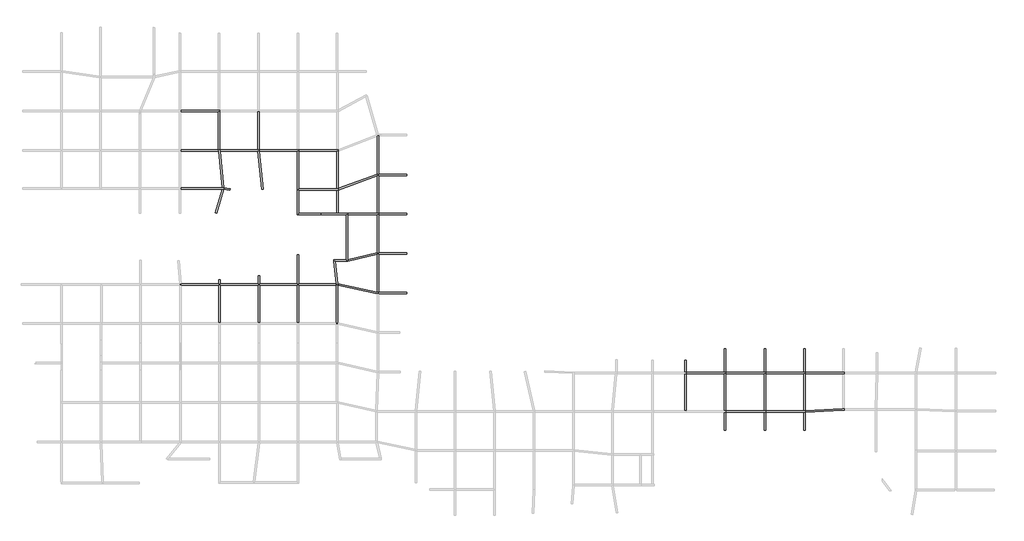
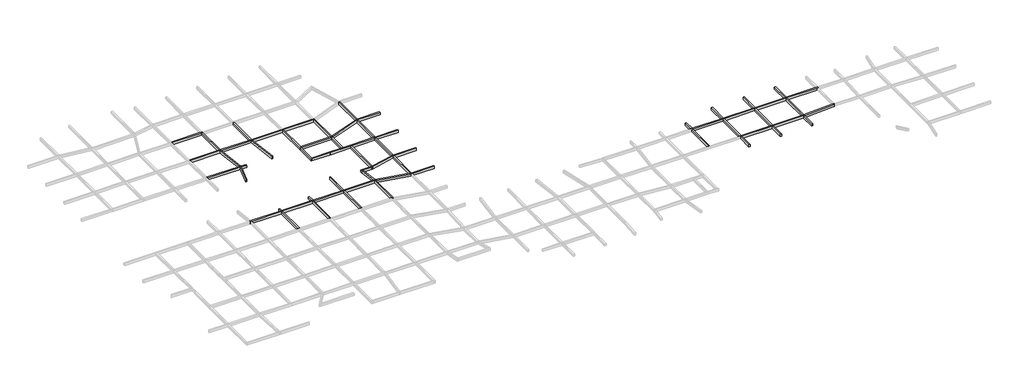
# One storey, part 5 of 8: 63 beams.
"""IFC4 building model written with IfcOpenShell, lengths in millimetres."""

from ifc_helpers import new_model, si_unit, frame, origin, place, context, project, spatial, polyline, outline, extrude, faceted_brep, element, save

model = new_model("IFC4")

# Units and contexts
model_context = context("Model", 3, world=origin())
ifc_project = project(units=[si_unit("LENGTHUNIT", "METRE", prefix="MILLI")], contexts=[model_context])

# Site, building, storey
site = spatial("IfcSite", under=ifc_project)
building = spatial("IfcBuilding", under=site)
storey = spatial("IfcBuildingStorey", under=building, Name="层高", Elevation=3300.0)

# Beams
placement = place(None, origin())
element("IfcBeam", 1, ObjectType="混凝土 - 矩形梁 : KL_beam", at=placement, inside=storey, context=model_context, shape_type="Brep", body=[
    faceted_brep([(134334.403154, 87731.7102801, 3300.0), (134334.403154, 88015.281938, 3300.0), (134334.403154, 88031.7102801, 3300.0), (134032.8693125, 88031.7102801, 3300.0), (125748.8238729, 88031.7102801, 3300.0), (125748.8238729, 87731.7102801, 3300.0), (133999.7671497, 87731.7102801, 3300.0), (134189.0731521, 87731.7102801, 3300.0), (134334.403154, 87731.7102801, 2700.0), (125748.8238729, 87731.7102801, 2700.0), (133999.7671497, 87731.7102801, 2700.0), (134189.0731521, 87731.7102801, 2700.0), (134334.403154, 88031.7102801, 2700.0), (134334.403154, 88015.281938, 2700.0), (125748.8238729, 88031.7102801, 2700.0), (134032.8693125, 88031.7102801, 2700.0)], [[[0, 1, 2, 3, 4, 5, 6, 7]], [[8, 0, 7, 6, 5, 9, 10, 11]], [[12, 13, 8, 11, 10, 9, 14, 15]], [[2, 12, 15, 14, 4, 3]], [[5, 4, 14, 9]], [[2, 1, 0, 8, 13, 12]]]),
])
element("IfcBeam", 2, ObjectType="混凝土 - 矩形梁 : KL_beam", at=placement, inside=storey, context=model_context, shape_type="Brep", body=[
    faceted_brep([(133564.8960768, 95631.7102801, 3300.0), (133548.8238805, 95631.7102801, 3300.0), (133263.3622352, 95631.7102801, 3300.0), (133293.7375146, 95331.7102801, 3300.0), (134032.8693125, 88031.7102801, 3300.0), (134334.403154, 88031.7102801, 3300.0), (133595.2713562, 95331.7102801, 3300.0), (133263.3622352, 95631.7102801, 2700.0), (133293.7375146, 95331.7102801, 2700.0), (134032.8693125, 88031.7102801, 2700.0), (133548.8238805, 95631.7102801, 2700.0), (133564.8960768, 95631.7102801, 2700.0), (133595.2713562, 95331.7102801, 2700.0), (134334.403154, 88031.7102801, 2700.0)], [[[0, 1, 2, 3, 4, 5, 6]], [[2, 7, 8, 9, 4, 3]], [[7, 10, 11, 12, 13, 9, 8]], [[11, 0, 6, 5, 13, 12]], [[5, 4, 9, 13]], [[2, 1, 0, 11, 10, 7]]]),
])
element("IfcBeam", 3, ObjectType="混凝土 - 矩形梁 : KL_beam", at=placement, inside=storey, context=model_context, shape_type="Brep", body=[
    faceted_brep([(125748.8238728, 95631.7102801, 3300.0), (125748.8238728, 95331.7102801, 3300.0), (133293.7375146, 95331.7102801, 3300.0), (133263.3622352, 95631.7102801, 3300.0), (133248.8238805, 95631.7102801, 3300.0), (125748.8238728, 95331.7102801, 2700.0), (133293.7375146, 95331.7102801, 2700.0), (125748.8238728, 95631.7102801, 2700.0), (133248.8238805, 95631.7102801, 2700.0), (133263.3622352, 95631.7102801, 2700.0)], [[[0, 1, 2, 3, 4]], [[1, 5, 6, 2]], [[5, 7, 8, 9, 6]], [[7, 0, 4, 3, 9, 8]], [[1, 0, 7, 5]], [[3, 2, 6, 9]]]),
])
element("IfcBeam", 4, ObjectType="混凝土 - 矩形梁 : KL_beam", at=placement, inside=storey, context=model_context, shape_type="Brep", body=[
    faceted_brep([(133548.8238805, 103231.7102801, 3300.0), (133548.8238805, 103531.7102801, 3300.0), (133248.8238805, 103531.7102801, 3300.0), (125748.8238726, 103531.7102801, 3300.0), (125748.8238726, 103231.7102801, 3300.0), (133248.8238805, 103231.7102801, 3300.0), (133548.8238805, 103231.7102801, 2700.0), (125748.8238726, 103231.7102801, 2700.0), (133248.8238805, 103231.7102801, 2700.0), (133548.8238805, 103531.7102801, 2700.0), (125748.8238726, 103531.7102801, 2700.0), (133248.8238805, 103531.7102801, 2700.0)], [[[0, 1, 2, 3, 4, 5]], [[6, 0, 5, 4, 7, 8]], [[9, 6, 8, 7, 10, 11]], [[1, 9, 11, 10, 3, 2]], [[4, 3, 10, 7]], [[1, 0, 6, 9]]]),
])
element("IfcBeam", 5, ObjectType="混凝土 - 矩形梁 : KL_beam", at=placement, inside=storey, context=model_context, shape_type="Brep", body=[
    faceted_brep([(133548.8238805, 103231.7102801, 3300.0), (133248.8238805, 103231.7102801, 3300.0), (133248.8238805, 95631.7102801, 3300.0), (133263.3622352, 95631.7102801, 3300.0), (133548.8238805, 95631.7102801, 3300.0), (133248.8238805, 103231.7102801, 2700.0), (133248.8238805, 95631.7102801, 2700.0), (133548.8238805, 103231.7102801, 2700.0), (133548.8238805, 95631.7102801, 2700.0), (133263.3622352, 95631.7102801, 2700.0)], [[[0, 1, 2, 3, 4]], [[1, 5, 6, 2]], [[5, 7, 8, 9, 6]], [[7, 0, 4, 8]], [[1, 0, 7, 5]], [[4, 3, 2, 6, 9, 8]]]),
])
element("IfcBeam", 6, ObjectType="混凝土 - 矩形梁 : KL_beam", at=placement, inside=storey, context=model_context, shape_type="Brep", body=[
    faceted_brep([(133564.8960768, 95631.7102801, 3300.0), (133595.2713562, 95331.7102801, 3300.0), (141163.7632738, 95331.7102801, 3300.0), (141465.4157577, 95331.7102801, 3300.0), (141448.8238805, 95489.571447, 3300.0), (141433.8844871, 95631.7102801, 3300.0), (141148.8238805, 95631.7102801, 3300.0), (133595.2713562, 95331.7102801, 2700.0), (141163.7632738, 95331.7102801, 2700.0), (141465.4157577, 95331.7102801, 2700.0), (133564.8960768, 95631.7102801, 2700.0), (141148.8238805, 95631.7102801, 2700.0), (141433.8844871, 95631.7102801, 2700.0), (141448.8238805, 95489.571447, 2700.0)], [[[0, 1, 2, 3, 4, 5, 6]], [[1, 7, 8, 9, 3, 2]], [[7, 10, 11, 12, 13, 9, 8]], [[10, 0, 6, 5, 12, 11]], [[1, 0, 10, 7]], [[5, 4, 3, 9, 13, 12]]]),
])
element("IfcBeam", 7, ObjectType="混凝土 - 矩形梁 : KL_beam", at=placement, inside=storey, context=model_context, shape_type="Brep", body=[
    faceted_brep([(135608.9251063, 87848.8786772, 3300.0), (135570.0863411, 87551.4033835, 3300.0), (135570.0863411, 87551.4033835, 2700.0), (135608.9251063, 87848.8786772, 2700.0), (134334.403154, 88015.281938, 3300.0), (134334.403154, 87731.7102801, 3300.0), (134189.0731521, 87731.7102801, 3300.0), (134307.4261, 87716.2579637, 3300.0), (134189.0731521, 87731.7102801, 2700.0), (134307.4261, 87716.2579637, 2700.0), (134334.403154, 87731.7102801, 2700.0), (134334.403154, 88015.281938, 2700.0)], [[[0, 1, 2, 3]], [[1, 0, 4, 5, 6, 7]], [[2, 1, 7, 6, 8, 9]], [[3, 2, 9, 8, 10, 11]], [[0, 3, 11, 4]], [[5, 10, 8, 6]], [[10, 5, 4, 11]]]),
])
element("IfcBeam", 8, ObjectType="混凝土 - 矩形梁 : KL_beam", at=placement, inside=storey, context=model_context, shape_type="SweptSolid", body=[
    extrude(outline(polyline([(142263.3241783, 87740.1187657), (141964.9676097, 87708.7602268), (141163.7632738, 95331.7102801), (141465.4157577, 95331.7102801), (142263.3241783, 87740.1187657)])), frame((0.0, 0.0, 2700.0), z_axis=(0.0, 0.0, 1.0), x_axis=(1.0, 0.0, 0.0)), (0.0, 0.0, 1.0), 600.0),
])
element("IfcBeam", 9, ObjectType="混凝土 - 矩形梁 : KL_beam", at=placement, inside=storey, context=model_context, shape_type="Brep", body=[
    faceted_brep([(132928.4176001, 82907.0838029, 3300.0), (132640.0390913, 82989.7750097, 3300.0), (132640.0390913, 82989.7750097, 2700.0), (132928.4176001, 82907.0838029, 2700.0), (134307.4261, 87716.2579637, 3300.0), (134189.0731521, 87731.7102801, 3300.0), (134063.2445918, 87731.7102801, 3300.0), (133999.7671497, 87731.7102801, 3300.0), (133999.7671497, 87731.7102801, 2700.0), (134063.2445918, 87731.7102801, 2700.0), (134189.0731521, 87731.7102801, 2700.0), (134307.4261, 87716.2579637, 2700.0)], [[[0, 1, 2, 3]], [[1, 0, 4, 5, 6, 7]], [[2, 1, 7, 8]], [[3, 2, 8, 9, 10, 11]], [[0, 3, 11, 4]], [[8, 7, 6, 5, 10, 9]], [[5, 4, 11, 10]]]),
])
element("IfcBeam", 10, ObjectType="混凝土 - 矩形梁 : KL_beam", at=placement, inside=storey, context=model_context, shape_type="Brep", body=[
    faceted_brep([(141448.8238805, 103231.7102801, 3300.0), (141148.8238805, 103231.7102801, 3300.0), (141148.8238805, 95631.7102801, 3300.0), (141433.8844871, 95631.7102801, 3300.0), (141448.8238805, 95489.571447, 3300.0), (141448.8238805, 95631.7102801, 3300.0), (141148.8238805, 103231.7102801, 2700.0), (141148.8238805, 95631.7102801, 2700.0), (141448.8238805, 103231.7102801, 2700.0), (141448.8238805, 95631.7102801, 2700.0), (141448.8238805, 95489.571447, 2700.0), (141433.8844871, 95631.7102801, 2700.0)], [[[0, 1, 2, 3, 4, 5]], [[1, 6, 7, 2]], [[6, 8, 9, 10, 11, 7]], [[8, 0, 5, 4, 10, 9]], [[1, 0, 8, 6]], [[11, 3, 2, 7]], [[3, 11, 10, 4]]]),
])
element("IfcBeam", 11, ObjectType="混凝土 - 矩形梁 : KL_beam", at=placement, inside=storey, context=model_context, shape_type="Brep", body=[
    faceted_brep([(149348.8238805, 95331.7102801, 3300.0), (149348.8238805, 95631.7102801, 3300.0), (149048.8238805, 95631.7102801, 3300.0), (141448.8238805, 95631.7102801, 3300.0), (141448.8238805, 95489.571447, 3300.0), (141465.4157577, 95331.7102801, 3300.0), (149048.8238805, 95331.7102801, 3300.0), (141465.4157577, 95331.7102801, 2700.0), (149048.8238805, 95331.7102801, 2700.0), (149348.8238805, 95331.7102801, 2700.0), (149348.8238805, 95631.7102801, 2700.0), (141448.8238805, 95489.571447, 2700.0), (141448.8238805, 95631.7102801, 2700.0), (149048.8238805, 95631.7102801, 2700.0)], [[[0, 1, 2, 3, 4, 5, 6]], [[5, 7, 8, 9, 0, 6]], [[10, 9, 8, 7, 11, 12, 13]], [[1, 10, 13, 12, 3, 2]], [[7, 5, 4, 11]], [[4, 3, 12, 11]], [[1, 0, 9, 10]]]),
])
element("IfcBeam", 12, ObjectType="混凝土 - 矩形梁 : KL_beam", at=placement, inside=storey, context=model_context, shape_type="Brep", body=[
    faceted_brep([(149048.8238805, 87550.0782767, 3300.0), (149348.8238805, 87550.0782767, 3300.0), (149348.8238805, 87850.0782767, 3300.0), (149348.8238805, 95331.7102801, 3300.0), (149048.8238805, 95331.7102801, 3300.0), (149048.8238805, 87550.0782767, 2700.0), (149048.8238805, 95331.7102801, 2700.0), (149348.8238805, 87550.0782767, 2700.0), (149348.8238805, 95331.7102801, 2700.0), (149348.8238805, 87850.0782767, 2700.0)], [[[0, 1, 2, 3, 4]], [[5, 0, 4, 6]], [[7, 5, 6, 8, 9]], [[1, 7, 9, 8, 3, 2]], [[4, 3, 8, 6]], [[1, 0, 5, 7]]]),
])
element("IfcBeam", 13, ObjectType="混凝土 - 矩形梁 : KL_beam", at=placement, inside=storey, context=model_context, shape_type="Brep", body=[
    faceted_brep([(157248.8238805, 95331.7102801, 3300.0), (157248.8238805, 95378.6181363, 3300.0), (157248.8238805, 95631.7102801, 3300.0), (156948.8238805, 95631.7102801, 3300.0), (149348.8238805, 95631.7102801, 3300.0), (149348.8238805, 95331.7102801, 3300.0), (156948.8238805, 95331.7102801, 3300.0), (157248.8238805, 95331.7102801, 2700.0), (149348.8238805, 95331.7102801, 2700.0), (156948.8238805, 95331.7102801, 2700.0), (157248.8238805, 95631.7102801, 2700.0), (157248.8238805, 95378.6181363, 2700.0), (149348.8238805, 95631.7102801, 2700.0), (156948.8238805, 95631.7102801, 2700.0)], [[[0, 1, 2, 3, 4, 5, 6]], [[7, 0, 6, 5, 8, 9]], [[10, 11, 7, 9, 8, 12, 13]], [[2, 10, 13, 12, 4, 3]], [[5, 4, 12, 8]], [[2, 1, 0, 7, 11, 10]]]),
])
element("IfcBeam", 14, ObjectType="混凝土 - 矩形梁 : KL_beam", at=placement, inside=storey, context=model_context, shape_type="Brep", body=[
    faceted_brep([(157248.8238805, 87550.0782767, 3300.0), (157248.8238805, 87595.0471459, 3300.0), (157248.8238805, 87850.0782767, 3300.0), (156948.8238805, 87850.0782767, 3300.0), (149348.8238805, 87850.0782767, 3300.0), (149348.8238805, 87550.0782767, 3300.0), (156948.8238805, 87550.0782767, 3300.0), (157248.8238805, 87550.0782767, 2700.0), (149348.8238805, 87550.0782767, 2700.0), (156948.8238805, 87550.0782767, 2700.0), (157248.8238805, 87850.0782767, 2700.0), (157248.8238805, 87595.0471459, 2700.0), (149348.8238805, 87850.0782767, 2700.0), (156948.8238805, 87850.0782767, 2700.0)], [[[0, 1, 2, 3, 4, 5, 6]], [[7, 0, 6, 5, 8, 9]], [[10, 11, 7, 9, 8, 12, 13]], [[2, 10, 13, 12, 4, 3]], [[5, 4, 12, 8]], [[2, 1, 0, 7, 11, 10]]]),
])
element("IfcBeam", 15, ObjectType="混凝土 - 矩形梁 : KL_beam", at=placement, inside=storey, context=model_context, shape_type="Brep", body=[
    faceted_brep([(157248.8238805, 95331.7102801, 3300.0), (156948.8238805, 95331.7102801, 3300.0), (156948.8238805, 87850.0782767, 3300.0), (157248.8238805, 87850.0782767, 3300.0), (157248.8238805, 87914.3004777, 3300.0), (156948.8238805, 95331.7102801, 2700.0), (156948.8238805, 87850.0782767, 2700.0), (157248.8238805, 95331.7102801, 2700.0), (157248.8238805, 87914.3004777, 2700.0), (157248.8238805, 87850.0782767, 2700.0)], [[[0, 1, 2, 3, 4]], [[1, 5, 6, 2]], [[5, 7, 8, 9, 6]], [[7, 0, 4, 3, 9, 8]], [[1, 0, 7, 5]], [[3, 2, 6, 9]]]),
])
element("IfcBeam", 16, ObjectType="混凝土 - 矩形梁 : KL_beam", at=placement, inside=storey, context=model_context, shape_type="Brep", body=[
    faceted_brep([(149048.8238805, 82650.0782767, 3300.0), (149348.8238805, 82650.0782767, 3300.0), (149348.8238805, 82950.0782767, 3300.0), (149348.8238805, 87550.0782767, 3300.0), (149048.8238805, 87550.0782767, 3300.0), (149048.8238805, 82650.0782767, 2700.0), (149048.8238805, 87550.0782767, 2700.0), (149348.8238805, 82650.0782767, 2700.0), (149348.8238805, 87550.0782767, 2700.0), (149348.8238805, 82950.0782767, 2700.0)], [[[0, 1, 2, 3, 4]], [[5, 0, 4, 6]], [[7, 5, 6, 8, 9]], [[1, 7, 9, 8, 3, 2]], [[4, 3, 8, 6]], [[1, 0, 5, 7]]]),
])
element("IfcBeam", 17, ObjectType="混凝土 - 矩形梁 : KL_beam", at=placement, inside=storey, context=model_context, shape_type="SweptSolid", body=[
    extrude(outline(polyline([(153790.5556896, 82950.0782767), (153790.5556896, 82650.0782767), (149348.8238805, 82650.0782767), (149348.8238805, 82950.0782767), (153790.5556896, 82950.0782767)])), frame((0.0, 0.0, 2700.0), z_axis=(0.0, 0.0, 1.0), x_axis=(1.0, 0.0, 0.0)), (0.0, 0.0, 1.0), 600.0),
])
element("IfcBeam", 18, ObjectType="混凝土 - 矩形梁 : KL_beam", at=placement, inside=storey, context=model_context, shape_type="Brep", body=[
    faceted_brep([(153790.5556896, 82950.0782767, 3300.0), (153790.5556896, 82650.0782767, 3300.0), (158923.8473255, 82650.0782767, 3300.0), (159223.8473255, 82650.0782767, 3300.0), (159223.8473255, 82950.0782767, 3300.0), (157248.8238805, 82950.0782767, 3300.0), (156948.8238805, 82950.0782767, 3300.0), (153790.5556896, 82650.0782767, 2700.0), (158923.8473255, 82650.0782767, 2700.0), (159223.8473255, 82650.0782767, 2700.0), (153790.5556896, 82950.0782767, 2700.0), (156948.8238805, 82950.0782767, 2700.0), (157248.8238805, 82950.0782767, 2700.0), (159223.8473255, 82950.0782767, 2700.0)], [[[0, 1, 2, 3, 4, 5, 6]], [[1, 7, 8, 9, 3, 2]], [[7, 10, 11, 12, 13, 9, 8]], [[10, 0, 6, 5, 4, 13, 12, 11]], [[0, 10, 7, 1]], [[4, 3, 9, 13]]]),
])
element("IfcBeam", 19, ObjectType="混凝土 - 矩形梁 : KL_beam", at=placement, inside=storey, context=model_context, shape_type="SweptSolid", body=[
    extrude(outline(polyline([(156948.8238805, 87550.0782767), (157248.8238805, 87550.0782767), (157248.8238805, 82950.0782767), (156948.8238805, 82950.0782767), (156948.8238805, 87550.0782767)])), frame((0.0, 0.0, 2700.0), z_axis=(0.0, 0.0, 1.0), x_axis=(1.0, 0.0, 0.0)), (0.0, 0.0, 1.0), 600.0),
])
element("IfcBeam", 20, ObjectType="混凝土 - 矩形梁 : KL_beam", at=placement, inside=storey, context=model_context, shape_type="Brep", body=[
    faceted_brep([(157248.8238805, 87595.0471459, 3300.0), (165070.973591, 90442.0768085, 3300.0), (165206.6294664, 90491.4515093, 3300.0), (165153.7313721, 90791.4515093, 3300.0), (165070.973591, 90761.3301403, 3300.0), (157248.8238805, 87914.3004777, 3300.0), (157248.8238805, 87850.0782767, 3300.0), (157248.8238805, 87595.0471459, 2700.0), (165070.973591, 90442.0768085, 2700.0), (165206.6294664, 90491.4515093, 2700.0), (157248.8238805, 87850.0782767, 2700.0), (157248.8238805, 87914.3004777, 2700.0), (165070.973591, 90761.3301403, 2700.0), (165153.7313721, 90791.4515093, 2700.0)], [[[0, 1, 2, 3, 4, 5, 6]], [[2, 1, 0, 7, 8, 9]], [[9, 8, 7, 10, 11, 12, 13]], [[5, 4, 3, 13, 12, 11]], [[7, 0, 6, 5, 11, 10]], [[3, 2, 9, 13]]]),
])
element("IfcBeam", 21, ObjectType="混凝土 - 矩形梁 : KL_beam", at=placement, inside=storey, context=model_context, shape_type="Brep", body=[
    faceted_brep([(170973.5021549, 90791.4515093, 3300.0), (170973.5021549, 90491.4515093, 3300.0), (170973.5021549, 90491.4515093, 2700.0), (170973.5021549, 90791.4515093, 2700.0), (165370.973591, 90791.4515093, 3300.0), (165153.7313721, 90791.4515093, 3300.0), (165206.6294664, 90491.4515093, 3300.0), (165370.973591, 90491.4515093, 3300.0), (165206.6294664, 90491.4515093, 2700.0), (165370.973591, 90491.4515093, 2700.0), (165153.7313721, 90791.4515093, 2700.0), (165370.973591, 90791.4515093, 2700.0)], [[[0, 1, 2, 3]], [[1, 0, 4, 5, 6, 7]], [[2, 1, 7, 6, 8, 9]], [[3, 2, 9, 8, 10, 11]], [[0, 3, 11, 10, 5, 4]], [[5, 10, 8, 6]]]),
])
element("IfcBeam", 22, ObjectType="混凝土 - 矩形梁 : KL_beam", at=placement, inside=storey, context=model_context, shape_type="SweptSolid", body=[
    extrude(outline(polyline([(165070.973591, 98381.2600869), (165248.7744478, 98449.5114412), (165370.973591, 98449.5114412), (165370.973591, 90791.4515093), (165153.7313721, 90791.4515093), (165070.973591, 90761.3301403), (165070.973591, 98381.2600869)])), frame((0.0, 0.0, 2700.0), z_axis=(0.0, 0.0, 1.0), x_axis=(1.0, 0.0, 0.0)), (0.0, 0.0, 1.0), 600.0),
])
element("IfcBeam", 23, ObjectType="混凝土 - 矩形梁 : KL_beam", at=placement, inside=storey, context=model_context, shape_type="Brep", body=[
    faceted_brep([(165370.973591, 82650.0782767, 3300.0), (165370.973591, 82950.0782767, 3300.0), (165070.973591, 82950.0782767, 3300.0), (159223.8473255, 82950.0782767, 3300.0), (159223.8473255, 82650.0782767, 3300.0), (165070.973591, 82650.0782767, 3300.0), (165370.973591, 82650.0782767, 2700.0), (159223.8473255, 82650.0782767, 2700.0), (165070.973591, 82650.0782767, 2700.0), (165370.973591, 82950.0782767, 2700.0), (159223.8473255, 82950.0782767, 2700.0), (165070.973591, 82950.0782767, 2700.0)], [[[0, 1, 2, 3, 4, 5]], [[6, 0, 5, 4, 7, 8]], [[9, 6, 8, 7, 10, 11]], [[1, 9, 11, 10, 3, 2]], [[1, 0, 6, 9]], [[4, 3, 10, 7]]]),
])
element("IfcBeam", 24, ObjectType="混凝土 - 矩形梁 : KL_beam", at=placement, inside=storey, context=model_context, shape_type="SweptSolid", body=[
    extrude(outline(polyline([(170973.3987408, 82950.0782767), (170973.3987408, 82650.0782767), (165370.973591, 82650.0782767), (165370.973591, 82950.0782767), (170973.3987408, 82950.0782767)])), frame((0.0, 0.0, 2700.0), z_axis=(0.0, 0.0, 1.0), x_axis=(1.0, 0.0, 0.0)), (0.0, 0.0, 1.0), 600.0),
])
element("IfcBeam", 25, ObjectType="混凝土 - 矩形梁 : KL_beam", at=placement, inside=storey, context=model_context, shape_type="SweptSolid", body=[
    extrude(outline(polyline([(165370.973591, 82950.0782767), (165070.973591, 82950.0782767), (165070.973591, 90442.0768085), (165206.6294664, 90491.4515093), (165370.973591, 90491.4515093), (165370.973591, 82950.0782767)])), frame((0.0, 0.0, 2700.0), z_axis=(0.0, 0.0, 1.0), x_axis=(1.0, 0.0, 0.0)), (0.0, 0.0, 1.0), 600.0),
])
element("IfcBeam", 26, ObjectType="混凝土 - 矩形梁 : KL_beam", at=placement, inside=storey, context=model_context, shape_type="Brep", body=[
    faceted_brep([(158923.8473255, 73320.7628892, 3300.0), (159223.8473255, 73320.7628892, 3300.0), (159223.8473255, 73628.6541215, 3300.0), (159223.8473255, 82650.0782767, 3300.0), (158923.8473255, 82650.0782767, 3300.0), (158923.8473255, 73590.0782767, 3300.0), (158923.8473255, 73320.7628892, 2700.0), (158923.8473255, 82650.0782767, 2700.0), (158923.8473255, 73590.0782767, 2700.0), (159223.8473255, 73320.7628892, 2700.0), (159223.8473255, 82650.0782767, 2700.0), (159223.8473255, 73628.6541215, 2700.0)], [[[0, 1, 2, 3, 4, 5]], [[6, 0, 5, 4, 7, 8]], [[9, 6, 8, 7, 10, 11]], [[1, 9, 11, 10, 3, 2]], [[4, 3, 10, 7]], [[1, 0, 6, 9]]]),
])
element("IfcBeam", 27, ObjectType="混凝土 - 矩形梁 : KL_beam", at=placement, inside=storey, context=model_context, shape_type="Brep", body=[
    faceted_brep([(159223.8473255, 73320.7628892, 3300.0), (165070.973591, 74670.6783534, 3300.0), (165132.0320684, 74684.7748136, 3300.0), (165097.851386, 74984.7748136, 3300.0), (165070.973591, 74978.5695857, 3300.0), (159223.8473255, 73628.6541215, 3300.0), (159223.8473255, 73320.7628892, 2700.0), (165070.973591, 74670.6783534, 2700.0), (165132.0320684, 74684.7748136, 2700.0), (159223.8473255, 73628.6541215, 2700.0), (165070.973591, 74978.5695857, 2700.0), (165097.851386, 74984.7748136, 2700.0)], [[[0, 1, 2, 3, 4, 5]], [[2, 1, 0, 6, 7, 8]], [[8, 7, 6, 9, 10, 11]], [[3, 11, 10, 9, 5, 4]], [[0, 5, 9, 6]], [[3, 2, 8, 11]]]),
])
element("IfcBeam", 28, ObjectType="混凝土 - 矩形梁 : KL_beam", at=placement, inside=storey, context=model_context, shape_type="Brep", body=[
    faceted_brep([(170973.3828089, 74984.7748136, 3300.0), (170973.3828089, 74684.7748136, 3300.0), (170973.3828089, 74684.7748136, 2700.0), (170973.3828089, 74984.7748136, 2700.0), (165370.973591, 74984.7748136, 3300.0), (165097.851386, 74984.7748136, 3300.0), (165132.0320684, 74684.7748136, 3300.0), (165370.973591, 74684.7748136, 3300.0), (165132.0320684, 74684.7748136, 2700.0), (165370.973591, 74684.7748136, 2700.0), (165097.851386, 74984.7748136, 2700.0), (165370.973591, 74984.7748136, 2700.0)], [[[0, 1, 2, 3]], [[1, 0, 4, 5, 6, 7]], [[2, 1, 7, 6, 8, 9]], [[3, 2, 9, 8, 10, 11]], [[0, 3, 11, 10, 5, 4]], [[5, 10, 8, 6]]]),
])
element("IfcBeam", 29, ObjectType="混凝土 - 矩形梁 : KL_beam", at=placement, inside=storey, context=model_context, shape_type="SweptSolid", body=[
    extrude(outline(polyline([(165070.973591, 82650.0782767), (165370.973591, 82650.0782767), (165370.973591, 74984.7748136), (165097.851386, 74984.7748136), (165070.973591, 74978.5695857), (165070.973591, 82650.0782767)])), frame((0.0, 0.0, 2700.0), z_axis=(0.0, 0.0, 1.0), x_axis=(1.0, 0.0, 0.0)), (0.0, 0.0, 1.0), 600.0),
])
element("IfcBeam", 30, ObjectType="混凝土 - 矩形梁 : KL_beam", at=placement, inside=storey, context=model_context, shape_type="Brep", body=[
    faceted_brep([(156358.7432126, 73290.0782767, 3300.0), (156660.9961603, 73290.0782767, 3300.0), (159090.9376668, 73290.0782767, 3300.0), (159223.8473255, 73320.7628892, 3300.0), (158923.8473255, 73320.7628892, 3300.0), (158923.8473255, 73559.3936642, 3300.0), (158923.8473255, 73590.0782767, 3300.0), (156358.7432126, 73590.0782767, 3300.0), (158923.8473255, 73590.0782767, 2700.0), (156358.7432126, 73590.0782767, 2700.0), (159090.9376668, 73290.0782767, 2700.0), (156660.9961603, 73290.0782767, 2700.0), (156358.7432126, 73290.0782767, 2700.0), (158923.8473255, 73559.3936642, 2700.0), (158923.8473255, 73320.7628892, 2700.0), (159223.8473255, 73320.7628892, 2700.0)], [[[0, 1, 2, 3, 4, 5, 6, 7]], [[7, 6, 8, 9]], [[10, 11, 12, 9, 8, 13, 14, 15]], [[2, 1, 0, 12, 11, 10]], [[3, 2, 10, 15]], [[4, 14, 13, 8, 6, 5]], [[14, 4, 3, 15]], [[0, 7, 9, 12]]]),
])
element("IfcBeam", 31, ObjectType="混凝土 - 矩形梁 : KL_beam", at=placement, inside=storey, context=model_context, shape_type="Brep", body=[
    faceted_brep([(156940.5822116, 68551.3799038, 3300.0), (157226.4248507, 68490.6221753, 3300.0), (157250.9349511, 68485.4123926, 3300.0), (157212.2674897, 68800.3335937, 3300.0), (156660.9961603, 73290.0782767, 3300.0), (156358.7432126, 73290.0782767, 3300.0), (156906.8806927, 68825.8567488, 3300.0), (156926.4248507, 68666.6823558, 3300.0), (156940.5822116, 68551.3799038, 2700.0), (156358.7432126, 73290.0782767, 2700.0), (156906.8806927, 68825.8567488, 2700.0), (156926.4248507, 68666.6823558, 2700.0), (157250.9349511, 68485.4123926, 2700.0), (157226.4248507, 68490.6221753, 2700.0), (156660.9961603, 73290.0782767, 2700.0), (157212.2674897, 68800.3335937, 2700.0)], [[[0, 1, 2, 3, 4, 5, 6, 7]], [[8, 0, 7, 6, 5, 9, 10, 11]], [[12, 13, 8, 11, 10, 9, 14, 15]], [[2, 12, 15, 14, 4, 3]], [[5, 4, 14, 9]], [[2, 1, 0, 8, 13, 12]]]),
])
element("IfcBeam", 32, ObjectType="混凝土 - 矩形梁 : KL_beam", at=placement, inside=storey, context=model_context, shape_type="Brep", body=[
    faceted_brep([(165277.0990615, 66779.3985459, 3300.0), (165308.6303321, 67079.3985459, 3300.0), (165070.973591, 67129.9140457, 3300.0), (157212.2674897, 68800.3335937, 3300.0), (157250.9349511, 68485.4123926, 3300.0), (165142.8646968, 66807.9309409, 3300.0), (165277.0990615, 66779.3985459, 2700.0), (157250.9349511, 68485.4123926, 2700.0), (165142.8646968, 66807.9309409, 2700.0), (165308.6303321, 67079.3985459, 2700.0), (157212.2674897, 68800.3335937, 2700.0), (165070.973591, 67129.9140457, 2700.0)], [[[0, 1, 2, 3, 4, 5]], [[6, 0, 5, 4, 7, 8]], [[9, 6, 8, 7, 10, 11]], [[1, 9, 11, 10, 3, 2]], [[4, 3, 10, 7]], [[1, 0, 6, 9]]]),
])
element("IfcBeam", 33, ObjectType="混凝土 - 矩形梁 : KL_beam", at=placement, inside=storey, context=model_context, shape_type="Brep", body=[
    faceted_brep([(170973.3442937, 67079.3985459, 3300.0), (170973.3442937, 66779.3985459, 3300.0), (170973.3442937, 66779.3985459, 2700.0), (170973.3442937, 67079.3985459, 2700.0), (165370.973591, 67079.3985459, 3300.0), (165308.6303321, 67079.3985459, 3300.0), (165277.0990615, 66779.3985459, 3300.0), (165442.8646968, 66779.3985459, 3300.0), (165277.0990615, 66779.3985459, 2700.0), (165442.8646968, 66779.3985459, 2700.0), (165308.6303321, 67079.3985459, 2700.0), (165370.973591, 67079.3985459, 2700.0)], [[[0, 1, 2, 3]], [[1, 0, 4, 5, 6, 7]], [[2, 1, 7, 6, 8, 9]], [[3, 2, 9, 8, 10, 11]], [[0, 3, 11, 10, 5, 4]], [[5, 10, 8, 6]]]),
])
element("IfcBeam", 34, ObjectType="混凝土 - 矩形梁 : KL_beam", at=placement, inside=storey, context=model_context, shape_type="SweptSolid", body=[
    extrude(outline(polyline([(165308.6303321, 67079.3985459), (165070.973591, 67129.9140457), (165070.973591, 74670.6783534), (165132.0320684, 74684.7748136), (165370.973591, 74684.7748136), (165370.973591, 67079.3985459), (165308.6303321, 67079.3985459)])), frame((0.0, 0.0, 2700.0), z_axis=(0.0, 0.0, 1.0), x_axis=(1.0, 0.0, 0.0)), (0.0, 0.0, 1.0), 600.0),
])
element("IfcBeam", 35, ObjectType="混凝土 - 矩形梁 : KL_beam", at=placement, inside=storey, context=model_context, shape_type="Brep", body=[
    faceted_brep([(156940.5822116, 68551.3799038, 3300.0), (156926.4248507, 68666.6823558, 3300.0), (156926.4248507, 68525.8567488, 3300.0), (156926.4248507, 61027.1438632, 3300.0), (156926.4248507, 60756.0063653, 3300.0), (157226.4248507, 60688.1226811, 3300.0), (157226.4248507, 60995.7071323, 3300.0), (157226.4248507, 68490.6221753, 3300.0), (156926.4248507, 68666.6823558, 2700.0), (156926.4248507, 68525.8567488, 2700.0), (156926.4248507, 61027.1438632, 2700.0), (156926.4248507, 60756.0063653, 2700.0), (156940.5822116, 68551.3799038, 2700.0), (157226.4248507, 68490.6221753, 2700.0), (157226.4248507, 60995.7071323, 2700.0), (157226.4248507, 60688.1226811, 2700.0)], [[[0, 1, 2, 3, 4, 5, 6, 7]], [[1, 8, 9, 10, 11, 4, 3, 2]], [[8, 12, 13, 14, 15, 11, 10, 9]], [[13, 7, 6, 5, 15, 14]], [[0, 12, 8, 1]], [[12, 0, 7, 13]], [[5, 4, 11, 15]]]),
])
element("IfcBeam", 36, ObjectType="混凝土 - 矩形梁 : KL_beam", at=placement, inside=storey, context=model_context, shape_type="Brep", body=[
    faceted_brep([(149026.4248507, 68825.8567488, 3300.0), (149026.4248507, 68525.8567488, 3300.0), (149326.4248507, 68525.8567488, 3300.0), (156926.4248507, 68525.8567488, 3300.0), (156926.4248507, 68666.6823558, 3300.0), (156906.8806927, 68825.8567488, 3300.0), (149326.4248507, 68825.8567488, 3300.0), (156906.8806927, 68825.8567488, 2700.0), (149326.4248507, 68825.8567488, 2700.0), (149026.4248507, 68825.8567488, 2700.0), (149026.4248507, 68525.8567488, 2700.0), (156926.4248507, 68666.6823558, 2700.0), (156926.4248507, 68525.8567488, 2700.0), (149326.4248507, 68525.8567488, 2700.0)], [[[0, 1, 2, 3, 4, 5, 6]], [[5, 7, 8, 9, 0, 6]], [[10, 9, 8, 7, 11, 12, 13]], [[1, 10, 13, 12, 3, 2]], [[7, 5, 4, 11]], [[4, 3, 12, 11]], [[1, 0, 9, 10]]]),
])
element("IfcBeam", 37, ObjectType="混凝土 - 矩形梁 : KL_beam", at=placement, inside=storey, context=model_context, shape_type="Brep", body=[
    faceted_brep([(141226.4248507, 68825.8567488, 3300.0), (141226.4248507, 68525.8567488, 3300.0), (141526.4248507, 68525.8567488, 3300.0), (149026.4248507, 68525.8567488, 3300.0), (149026.4248507, 68825.8567488, 3300.0), (141526.4248507, 68825.8567488, 3300.0), (141226.4248507, 68825.8567488, 2700.0), (149026.4248507, 68825.8567488, 2700.0), (141526.4248507, 68825.8567488, 2700.0), (141226.4248507, 68525.8567488, 2700.0), (149026.4248507, 68525.8567488, 2700.0), (141526.4248507, 68525.8567488, 2700.0)], [[[0, 1, 2, 3, 4, 5]], [[6, 0, 5, 4, 7, 8]], [[9, 6, 8, 7, 10, 11]], [[1, 9, 11, 10, 3, 2]], [[4, 3, 10, 7]], [[1, 0, 6, 9]]]),
])
element("IfcBeam", 38, ObjectType="混凝土 - 矩形梁 : KL_beam", at=placement, inside=storey, context=model_context, shape_type="Brep", body=[
    faceted_brep([(133326.4248507, 68825.8567488, 3300.0), (133326.4248507, 68525.8567488, 3300.0), (133626.4248507, 68525.8567488, 3300.0), (141226.4248507, 68525.8567488, 3300.0), (141226.4248507, 68825.8567488, 3300.0), (133626.4248507, 68825.8567488, 3300.0), (133326.4248507, 68825.8567488, 2700.0), (141226.4248507, 68825.8567488, 2700.0), (133626.4248507, 68825.8567488, 2700.0), (133326.4248507, 68525.8567488, 2700.0), (141226.4248507, 68525.8567488, 2700.0), (133626.4248507, 68525.8567488, 2700.0)], [[[0, 1, 2, 3, 4, 5]], [[6, 0, 5, 4, 7, 8]], [[9, 6, 8, 7, 10, 11]], [[1, 9, 11, 10, 3, 2]], [[1, 0, 6, 9]], [[4, 3, 10, 7]]]),
])
element("IfcBeam", 39, ObjectType="混凝土 - 矩形梁 : KL_beam", at=placement, inside=storey, context=model_context, shape_type="Brep", body=[
    faceted_brep([(125476.4248507, 68825.8567488, 3300.0), (125476.4248507, 68525.8567488, 3300.0), (125548.8240412, 68525.8567488, 3300.0), (125848.8240412, 68525.8567488, 3300.0), (133326.4248507, 68525.8567488, 3300.0), (133326.4248507, 68825.8567488, 3300.0), (125835.1476174, 68825.8567488, 3300.0), (125533.7755541, 68825.8567488, 3300.0), (125476.4248507, 68825.8567488, 2700.0), (133326.4248507, 68825.8567488, 2700.0), (125835.1476174, 68825.8567488, 2700.0), (125533.7755541, 68825.8567488, 2700.0), (125476.4248507, 68525.8567488, 2700.0), (133326.4248507, 68525.8567488, 2700.0), (125848.8240412, 68525.8567488, 2700.0), (125548.8240412, 68525.8567488, 2700.0)], [[[0, 1, 2, 3, 4, 5, 6, 7]], [[8, 0, 7, 6, 5, 9, 10, 11]], [[12, 8, 11, 10, 9, 13, 14, 15]], [[1, 12, 15, 14, 13, 4, 3, 2]], [[1, 0, 8, 12]], [[5, 4, 13, 9]]]),
])
element("IfcBeam", 40, ObjectType="混凝土 - 矩形梁 : KL_beam", at=placement, inside=storey, context=model_context, shape_type="SweptSolid", body=[
    extrude(outline(polyline([(149026.4248507, 68525.8567488), (149326.4248507, 68525.8567488), (149326.4248507, 61027.1438632), (149026.4248507, 61027.1438632), (149026.4248507, 68525.8567488)])), frame((0.0, 0.0, 2700.0), z_axis=(0.0, 0.0, 1.0), x_axis=(1.0, 0.0, 0.0)), (0.0, 0.0, 1.0), 600.0),
])
element("IfcBeam", 41, ObjectType="混凝土 - 矩形梁 : KL_beam", at=placement, inside=storey, context=model_context, shape_type="SweptSolid", body=[
    extrude(outline(polyline([(133326.4248507, 68525.8567488), (133626.4248507, 68525.8567488), (133626.4248507, 61027.1438632), (133326.4248507, 61027.1438632), (133326.4248507, 68525.8567488)])), frame((0.0, 0.0, 2700.0), z_axis=(0.0, 0.0, 1.0), x_axis=(1.0, 0.0, 0.0)), (0.0, 0.0, 1.0), 600.0),
])
element("IfcBeam", 42, ObjectType="混凝土 - 矩形梁 : KL_beam", at=placement, inside=storey, context=model_context, shape_type="SweptSolid", body=[
    extrude(outline(polyline([(141226.4248507, 68525.8567488), (141526.4248507, 68525.8567488), (141526.4248507, 61027.1438632), (141226.4248507, 61027.1438632), (141226.4248507, 68525.8567488)])), frame((0.0, 0.0, 2700.0), z_axis=(0.0, 0.0, 1.0), x_axis=(1.0, 0.0, 0.0)), (0.0, 0.0, 1.0), 600.0),
])
element("IfcBeam", 43, ObjectType="混凝土 - 矩形梁 : KL_beam", at=placement, inside=storey, context=model_context, shape_type="Brep", body=[
    faceted_brep([(234948.824042, 50816.8475615, 3300.0), (234948.824042, 51116.8475615, 3300.0), (234934.4881621, 51116.8475615, 3300.0), (234634.4881621, 51116.8475615, 3300.0), (227048.824042, 51116.8475615, 3300.0), (227048.824042, 50816.8475615, 3300.0), (234648.824042, 50816.8475615, 3300.0), (234948.824042, 50816.8475615, 2700.0), (227048.824042, 50816.8475615, 2700.0), (234648.824042, 50816.8475615, 2700.0), (234948.824042, 51116.8475615, 2700.0), (227048.824042, 51116.8475615, 2700.0), (234634.4881621, 51116.8475615, 2700.0), (234934.4881621, 51116.8475615, 2700.0)], [[[0, 1, 2, 3, 4, 5, 6]], [[7, 0, 6, 5, 8, 9]], [[10, 7, 9, 8, 11, 12, 13]], [[1, 10, 13, 12, 11, 4, 3, 2]], [[5, 4, 11, 8]], [[1, 0, 7, 10]]]),
])
element("IfcBeam", 44, ObjectType="混凝土 - 矩形梁 : KL_beam", at=placement, inside=storey, context=model_context, shape_type="SweptSolid", body=[
    extrude(outline(polyline([(226748.824042, 53516.2415345), (227048.824042, 53516.2415345), (227048.824042, 51116.8475615), (226748.824042, 51116.8475615), (226748.824042, 53516.2415345)])), frame((0.0, 0.0, 2700.0), z_axis=(0.0, 0.0, 1.0), x_axis=(1.0, 0.0, 0.0)), (0.0, 0.0, 1.0), 600.0),
])
element("IfcBeam", 45, ObjectType="混凝土 - 矩形梁 : KL_beam", at=placement, inside=storey, context=model_context, shape_type="SweptSolid", body=[
    extrude(outline(polyline([(234634.4881621, 55816.1792972), (234934.4881621, 55816.1792972), (234934.4881621, 51116.8475615), (234634.4881621, 51116.8475615), (234634.4881621, 55816.1792972)])), frame((0.0, 0.0, 2700.0), z_axis=(0.0, 0.0, 1.0), x_axis=(1.0, 0.0, 0.0)), (0.0, 0.0, 1.0), 600.0),
])
element("IfcBeam", 46, ObjectType="混凝土 - 矩形梁 : KL_beam", at=placement, inside=storey, context=model_context, shape_type="Brep", body=[
    faceted_brep([(242934.4881621, 50816.8475615, 3300.0), (242934.4881621, 51116.8475615, 3300.0), (242634.4881621, 51116.8475615, 3300.0), (234948.824042, 51116.8475615, 3300.0), (234948.824042, 50816.8475615, 3300.0), (242634.4881621, 50816.8475615, 3300.0), (242934.4881621, 50816.8475615, 2700.0), (234948.824042, 50816.8475615, 2700.0), (242634.4881621, 50816.8475615, 2700.0), (242934.4881621, 51116.8475615, 2700.0), (234948.824042, 51116.8475615, 2700.0), (242634.4881621, 51116.8475615, 2700.0)], [[[0, 1, 2, 3, 4, 5]], [[6, 0, 5, 4, 7, 8]], [[9, 6, 8, 7, 10, 11]], [[1, 9, 11, 10, 3, 2]], [[1, 0, 6, 9]], [[4, 3, 10, 7]]]),
])
element("IfcBeam", 47, ObjectType="混凝土 - 矩形梁 : KL_beam", at=placement, inside=storey, context=model_context, shape_type="Brep", body=[
    faceted_brep([(250834.4881621, 50816.8475615, 3300.0), (250834.4881621, 51116.8475615, 3300.0), (250534.4881621, 51116.8475615, 3300.0), (242934.4881621, 51116.8475615, 3300.0), (242934.4881621, 50816.8475615, 3300.0), (250534.4881621, 50816.8475615, 3300.0), (250834.4881621, 50816.8475615, 2700.0), (242934.4881621, 50816.8475615, 2700.0), (250534.4881621, 50816.8475615, 2700.0), (250834.4881621, 51116.8475615, 2700.0), (242934.4881621, 51116.8475615, 2700.0), (250534.4881621, 51116.8475615, 2700.0)], [[[0, 1, 2, 3, 4, 5]], [[6, 0, 5, 4, 7, 8]], [[9, 6, 8, 7, 10, 11]], [[1, 9, 11, 10, 3, 2]], [[1, 0, 6, 9]], [[4, 3, 10, 7]]]),
])
element("IfcBeam", 48, ObjectType="混凝土 - 矩形梁 : KL_beam", at=placement, inside=storey, context=model_context, shape_type="Brep", body=[
    faceted_brep([(258734.4881621, 50816.8475615, 3300.0), (258734.4881621, 51116.8475615, 3300.0), (258434.4881621, 51116.8475615, 3300.0), (250834.4881621, 51116.8475615, 3300.0), (250834.4881621, 50816.8475615, 3300.0), (258434.4881621, 50816.8475615, 3300.0), (258734.4881621, 50816.8475615, 2700.0), (250834.4881621, 50816.8475615, 2700.0), (258434.4881621, 50816.8475615, 2700.0), (258734.4881621, 51116.8475615, 2700.0), (250834.4881621, 51116.8475615, 2700.0), (258434.4881621, 51116.8475615, 2700.0)], [[[0, 1, 2, 3, 4, 5]], [[6, 0, 5, 4, 7, 8]], [[9, 6, 8, 7, 10, 11]], [[1, 9, 11, 10, 3, 2]], [[1, 0, 6, 9]], [[4, 3, 10, 7]]]),
])
element("IfcBeam", 49, ObjectType="混凝土 - 矩形梁 : KL_beam", at=placement, inside=storey, context=model_context, shape_type="SweptSolid", body=[
    extrude(outline(polyline([(250534.4881621, 55816.1792972), (250834.4881621, 55816.1792972), (250834.4881621, 51116.8475615), (250534.4881621, 51116.8475615), (250534.4881621, 55816.1792972)])), frame((0.0, 0.0, 2700.0), z_axis=(0.0, 0.0, 1.0), x_axis=(1.0, 0.0, 0.0)), (0.0, 0.0, 1.0), 600.0),
])
element("IfcBeam", 50, ObjectType="混凝土 - 矩形梁 : KL_beam", at=placement, inside=storey, context=model_context, shape_type="SweptSolid", body=[
    extrude(outline(polyline([(242634.4881621, 55816.1792972), (242934.4881621, 55816.1792972), (242934.4881621, 51116.8475615), (242634.4881621, 51116.8475615), (242634.4881621, 55816.1792972)])), frame((0.0, 0.0, 2700.0), z_axis=(0.0, 0.0, 1.0), x_axis=(1.0, 0.0, 0.0)), (0.0, 0.0, 1.0), 600.0),
])
element("IfcBeam", 51, ObjectType="混凝土 - 矩形梁 : KL_beam", at=placement, inside=storey, context=model_context, shape_type="SweptSolid", body=[
    extrude(outline(polyline([(133326.4248507, 69575.8567488), (133626.4248507, 69575.8567488), (133626.4248507, 68825.8567488), (133326.4248507, 68825.8567488), (133326.4248507, 69575.8567488)])), frame((0.0, 0.0, 2700.0), z_axis=(0.0, 0.0, 1.0), x_axis=(1.0, 0.0, 0.0)), (0.0, 0.0, 1.0), 600.0),
])
element("IfcBeam", 52, ObjectType="混凝土 - 矩形梁 : KL_beam", at=placement, inside=storey, context=model_context, shape_type="SweptSolid", body=[
    extrude(outline(polyline([(141226.4248507, 70400.0757628), (141526.4248507, 70400.0757628), (141526.4248507, 68825.8567488), (141226.4248507, 68825.8567488), (141226.4248507, 70400.0757628)])), frame((0.0, 0.0, 2700.0), z_axis=(0.0, 0.0, 1.0), x_axis=(1.0, 0.0, 0.0)), (0.0, 0.0, 1.0), 600.0),
])
element("IfcBeam", 53, ObjectType="混凝土 - 矩形梁 : KL_beam", at=placement, inside=storey, context=model_context, shape_type="SweptSolid", body=[
    extrude(outline(polyline([(149026.4248507, 74575.8567488), (149326.4248507, 74575.8567488), (149326.4248507, 68825.8567488), (149026.4248507, 68825.8567488), (149026.4248507, 74575.8567488)])), frame((0.0, 0.0, 2700.0), z_axis=(0.0, 0.0, 1.0), x_axis=(1.0, 0.0, 0.0)), (0.0, 0.0, 1.0), 600.0),
])
element("IfcBeam", 54, ObjectType="混凝土 - 矩形梁 : KL_beam", at=placement, inside=storey, context=model_context, shape_type="SweptSolid", body=[
    extrude(outline(polyline([(226748.824042, 50816.8475615), (227048.824042, 50816.8475615), (227048.824042, 43383.0583741), (226748.824042, 43383.0583741), (226748.824042, 50816.8475615)])), frame((0.0, 0.0, 2700.0), z_axis=(0.0, 0.0, 1.0), x_axis=(1.0, 0.0, 0.0)), (0.0, 0.0, 1.0), 600.0),
])
element("IfcBeam", 55, ObjectType="混凝土 - 矩形梁 : KL_beam", at=placement, inside=storey, context=model_context, shape_type="SweptSolid", body=[
    extrude(outline(polyline([(234648.824042, 50816.8475615), (234948.824042, 50816.8475615), (234948.824042, 43383.0583741), (234648.824042, 43383.0583741), (234648.824042, 50816.8475615)])), frame((0.0, 0.0, 2700.0), z_axis=(0.0, 0.0, 1.0), x_axis=(1.0, 0.0, 0.0)), (0.0, 0.0, 1.0), 600.0),
])
element("IfcBeam", 56, ObjectType="混凝土 - 矩形梁 : KL_beam", at=placement, inside=storey, context=model_context, shape_type="SweptSolid", body=[
    extrude(outline(polyline([(234948.824042, 39466.7058844), (234648.824042, 39466.7058844), (234648.824042, 43083.0583741), (234948.824042, 43083.0583741), (234948.824042, 39466.7058844)])), frame((0.0, 0.0, 2700.0), z_axis=(0.0, 0.0, 1.0), x_axis=(1.0, 0.0, 0.0)), (0.0, 0.0, 1.0), 600.0),
])
element("IfcBeam", 57, ObjectType="混凝土 - 矩形梁 : KL_beam", at=placement, inside=storey, context=model_context, shape_type="Brep", body=[
    faceted_brep([(242934.4881621, 43083.0583741, 3300.0), (242934.4881621, 43383.0583741, 3300.0), (242634.4881621, 43383.0583741, 3300.0), (234948.824042, 43383.0583741, 3300.0), (234948.824042, 43083.0583741, 3300.0), (242634.4881621, 43083.0583741, 3300.0), (242934.4881621, 43083.0583741, 2700.0), (234948.824042, 43083.0583741, 2700.0), (242634.4881621, 43083.0583741, 2700.0), (242934.4881621, 43383.0583741, 2700.0), (234948.824042, 43383.0583741, 2700.0), (242634.4881621, 43383.0583741, 2700.0)], [[[0, 1, 2, 3, 4, 5]], [[6, 0, 5, 4, 7, 8]], [[9, 6, 8, 7, 10, 11]], [[1, 9, 11, 10, 3, 2]], [[4, 3, 10, 7]], [[1, 0, 6, 9]]]),
])
element("IfcBeam", 58, ObjectType="混凝土 - 矩形梁 : KL_beam", at=placement, inside=storey, context=model_context, shape_type="Brep", body=[
    faceted_brep([(250834.4881621, 43083.0583741, 3300.0), (250834.4881621, 43090.7136891, 3300.0), (250834.4881621, 43383.0583741, 3300.0), (250534.4881621, 43383.0583741, 3300.0), (242934.4881621, 43383.0583741, 3300.0), (242934.4881621, 43083.0583741, 3300.0), (250534.4881621, 43083.0583741, 3300.0), (250834.4881621, 43083.0583741, 2700.0), (242934.4881621, 43083.0583741, 2700.0), (250534.4881621, 43083.0583741, 2700.0), (250834.4881621, 43383.0583741, 2700.0), (250834.4881621, 43090.7136891, 2700.0), (242934.4881621, 43383.0583741, 2700.0), (250534.4881621, 43383.0583741, 2700.0)], [[[0, 1, 2, 3, 4, 5, 6]], [[7, 0, 6, 5, 8, 9]], [[10, 11, 7, 9, 8, 12, 13]], [[2, 10, 13, 12, 4, 3]], [[5, 4, 12, 8]], [[2, 1, 0, 7, 11, 10]]]),
])
element("IfcBeam", 59, ObjectType="混凝土 - 矩形梁 : KL_beam", at=placement, inside=storey, context=model_context, shape_type="SweptSolid", body=[
    extrude(outline(polyline([(242634.4881621, 50816.8475615), (242934.4881621, 50816.8475615), (242934.4881621, 43383.0583741), (242634.4881621, 43383.0583741), (242634.4881621, 50816.8475615)])), frame((0.0, 0.0, 2700.0), z_axis=(0.0, 0.0, 1.0), x_axis=(1.0, 0.0, 0.0)), (0.0, 0.0, 1.0), 600.0),
])
element("IfcBeam", 60, ObjectType="混凝土 - 矩形梁 : KL_beam", at=placement, inside=storey, context=model_context, shape_type="SweptSolid", body=[
    extrude(outline(polyline([(242934.4881621, 39466.7058844), (242634.4881621, 39466.7058844), (242634.4881621, 43083.0583741), (242934.4881621, 43083.0583741), (242934.4881621, 39466.7058844)])), frame((0.0, 0.0, 2700.0), z_axis=(0.0, 0.0, 1.0), x_axis=(1.0, 0.0, 0.0)), (0.0, 0.0, 1.0), 600.0),
])
element("IfcBeam", 61, ObjectType="混凝土 - 矩形梁 : KL_beam", at=placement, inside=storey, context=model_context, shape_type="Brep", body=[
    faceted_brep([(250834.4881621, 50816.8475615, 3300.0), (250534.4881621, 50816.8475615, 3300.0), (250534.4881621, 43383.0583741, 3300.0), (250834.4881621, 43383.0583741, 3300.0), (250834.4881621, 43391.1253929, 3300.0), (250534.4881621, 50816.8475615, 2700.0), (250534.4881621, 43383.0583741, 2700.0), (250834.4881621, 50816.8475615, 2700.0), (250834.4881621, 43391.1253929, 2700.0), (250834.4881621, 43383.0583741, 2700.0)], [[[0, 1, 2, 3, 4]], [[1, 5, 6, 2]], [[5, 7, 8, 9, 6]], [[7, 0, 4, 3, 9, 8]], [[1, 0, 7, 5]], [[3, 2, 6, 9]]]),
])
element("IfcBeam", 62, ObjectType="混凝土 - 矩形梁 : KL_beam", at=placement, inside=storey, context=model_context, shape_type="SweptSolid", body=[
    extrude(outline(polyline([(250834.4881621, 39466.7058844), (250534.4881621, 39466.7058844), (250534.4881621, 43083.0583741), (250834.4881621, 43083.0583741), (250834.4881621, 39466.7058844)])), frame((0.0, 0.0, 2700.0), z_axis=(0.0, 0.0, 1.0), x_axis=(1.0, 0.0, 0.0)), (0.0, 0.0, 1.0), 600.0),
])
element("IfcBeam", 63, ObjectType="混凝土 - 矩形梁 : KL_beam", at=placement, inside=storey, context=model_context, shape_type="Brep", body=[
    faceted_brep([(250834.4881621, 43391.1253929, 3300.0), (250834.4881621, 43383.0583741, 3300.0), (250834.4881621, 43090.7136891, 3300.0), (258434.4881621, 43489.0128116, 3300.0), (258588.4160503, 43497.0798304, 3300.0), (258734.4881621, 43504.7351454, 3300.0), (258734.4881621, 43797.0798304, 3300.0), (258734.4881621, 43805.1468492, 3300.0), (258434.4881621, 43789.4245154, 3300.0), (250834.4881621, 43090.7136891, 2700.0), (258434.4881621, 43489.0128116, 2700.0), (258588.4160503, 43497.0798304, 2700.0), (258734.4881621, 43504.7351454, 2700.0), (250834.4881621, 43383.0583741, 2700.0), (250834.4881621, 43391.1253929, 2700.0), (258434.4881621, 43789.4245154, 2700.0), (258734.4881621, 43805.1468492, 2700.0), (258734.4881621, 43797.0798304, 2700.0)], [[[0, 1, 2, 3, 4, 5, 6, 7, 8]], [[2, 9, 10, 11, 12, 5, 4, 3]], [[9, 13, 14, 15, 16, 17, 12, 11, 10]], [[14, 0, 8, 7, 16, 15]], [[9, 2, 1, 0, 14, 13]], [[7, 6, 5, 12, 17, 16]]]),
])

save(model, "model.ifc")

# Revit data of these elements
# Type "混凝土 - 矩形梁 : KL_beam"
#   Length [instance default] = 1524 mm
#   b = 300 mm
#   h = 600 mm
#   Structural Material [instance default] = 混凝土 - 现场浇注混凝土
#   Assembly Code = ""
# Elements 1, 2, 3, 4, 5, 6, 7, 8, 9, 10, 11, 12, 13, 14, 15, 16, 17, 18, 19, 20, 21, 22, 23, 24, 25, 26, 27, 28, 29, 30, 31, 32, 33, 34, 35, 36, 37, 38, 39, 40, 41, 42, 43, 44, 45, 46, 47, 48, 49, 50, 51, 52, 53, 54, 55, 56, 57, 58, 59, 60, 61, 62, 63 (IfcBeam, "混凝土 - 矩形梁 : KL_beam")
#   Comments = ""
#   Structural Material = none
#   Phase Created = 新构造
# Materials
#   "混凝土 - 现场浇注混凝土": class "混凝土", colour RGB 192 192 192, transparency 0
